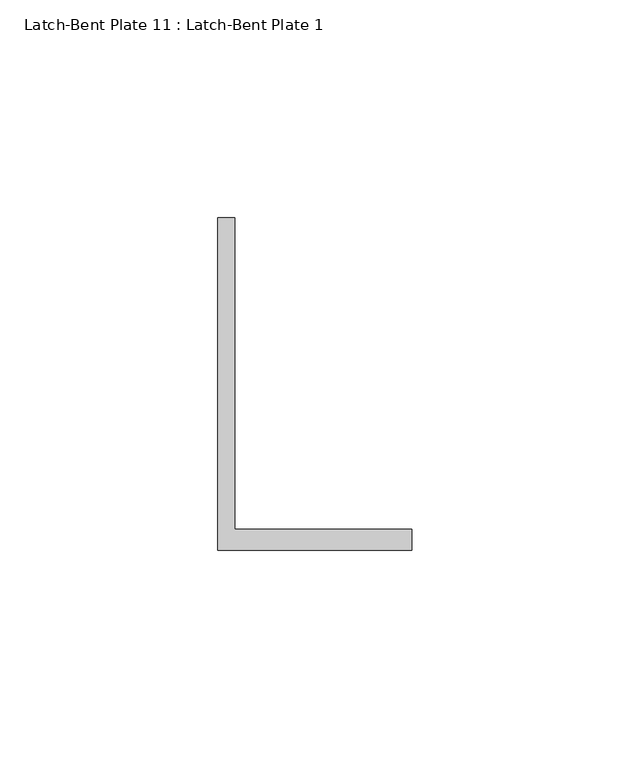
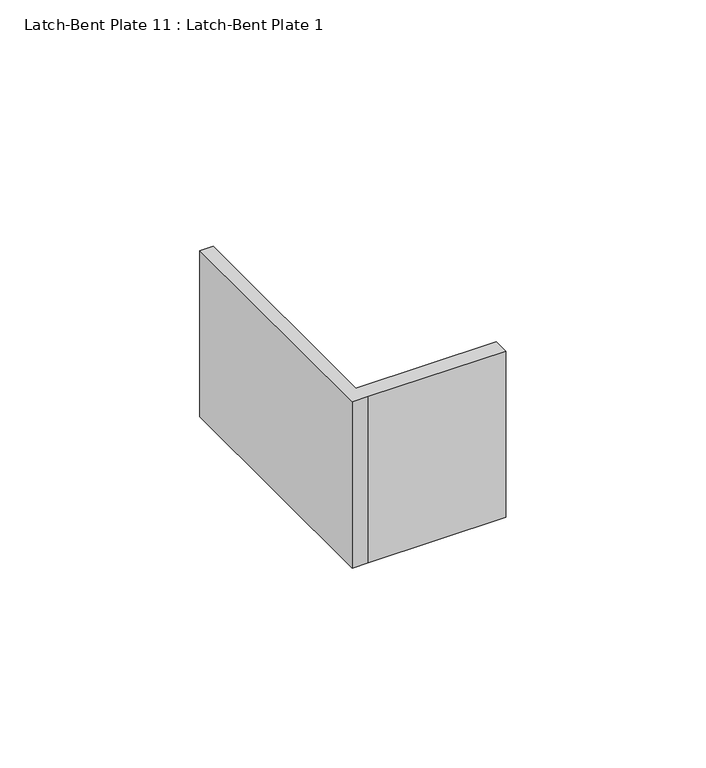
"""IFC4 building model written with IfcOpenShell, lengths in millimetres: proxy geometry, Latch-Bent Plate 11 : Latch-Bent Plate 1."""

from ifc_helpers import new_model, si_unit, frame, origin, place, context, project, spatial, polyline, outline, extrude, source, transform, mapped, element, save


def latch_bent_plate_11_latch_bent_plate_1_9e542a81(model_context):
    return source(origin(), model_context, "Body", "SweptSolid", [
        extrude(outline(polyline([(587327.0060739, -535201.5663841), (587322.2435739, -535201.5663841), (587322.2435739, -535125.3663841), (587326.1141748, -535125.3663841), (587326.1141748, -535196.8038841), (587366.6808739, -535196.8038841), (587366.6808739, -535201.5663841), (587327.0060739, -535201.5663841)])), frame((0.0, 0.0, 1041.4), z_axis=(0.0, 0.0, 1.0), x_axis=(1.0, 0.0, 0.0)), (0.0, 0.0, 1.0), 50.8),
    ])


if __name__ == "__main__":
    model = new_model("IFC4")
    model_context = context("Model", 3, world=origin())
    ifc_project = project(units=[si_unit("LENGTHUNIT", "METRE", prefix="MILLI")], contexts=[model_context])
    site = spatial("IfcSite", under=ifc_project)
    building = spatial("IfcBuilding", under=site)
    placement = place(None, origin())
    latch_bent_plate_11_latch_bent_plate_1_shape = latch_bent_plate_11_latch_bent_plate_1_9e542a81(model_context)
    element("IfcBuildingElementProxy", 1, Name="Latch-Bent Plate 11 : Latch-Bent Plate 1", ObjectType="Latch-Bent Plate 11 : Latch-Bent Plate 1", at=placement, inside=building, context=model_context, shape_type="MappedRepresentation", body=[
        mapped(latch_bent_plate_11_latch_bent_plate_1_shape, transform((0.0, 0.0, 0.0), x_axis=(1.0, 0.0, 0.0), y_axis=(0.0, 1.0, 0.0), z_axis=(0.0, 0.0, 1.0))),
    ])
    save(model, "model.ifc")

# Revit data of these elements
# Element 1 (IfcBuildingElementProxy, "Latch-Bent Plate 11 : Latch-Bent Plate 1")
#   Materials on its faces: "GALV. GATE LATCH"
# Materials
#   "GALV. GATE LATCH": class "Metal", colour RGB 189 187 185, transparency 0, Description = "Carbon steel", Cost = 0
